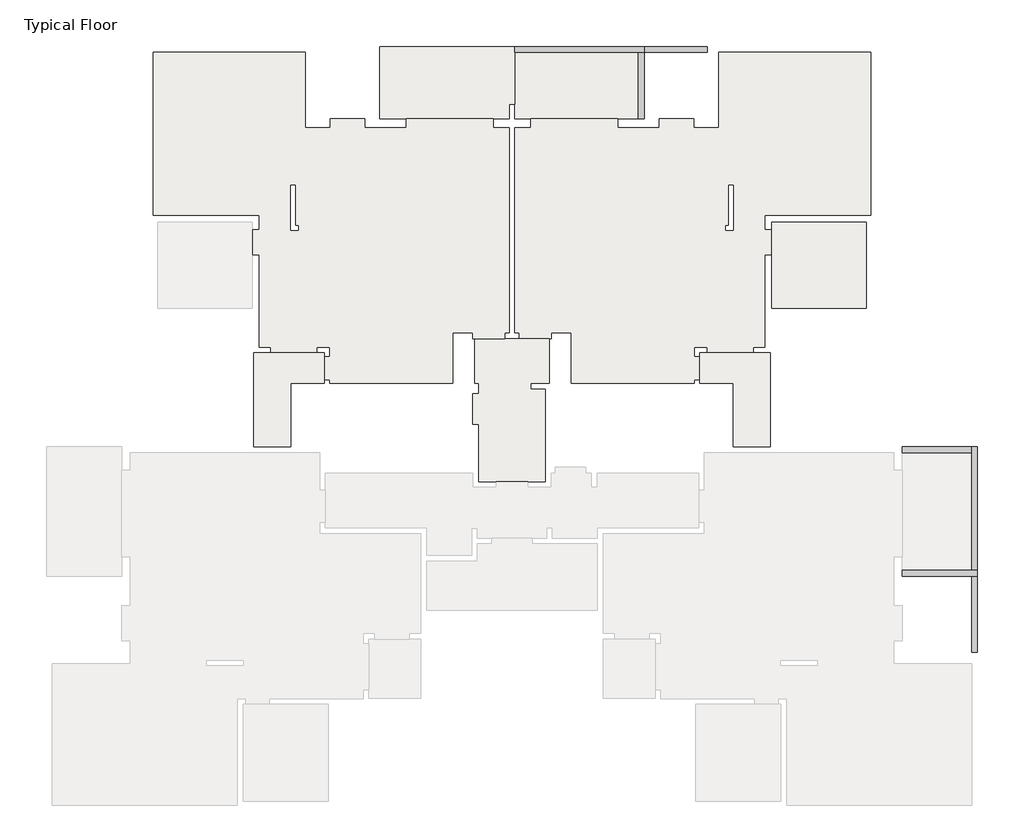
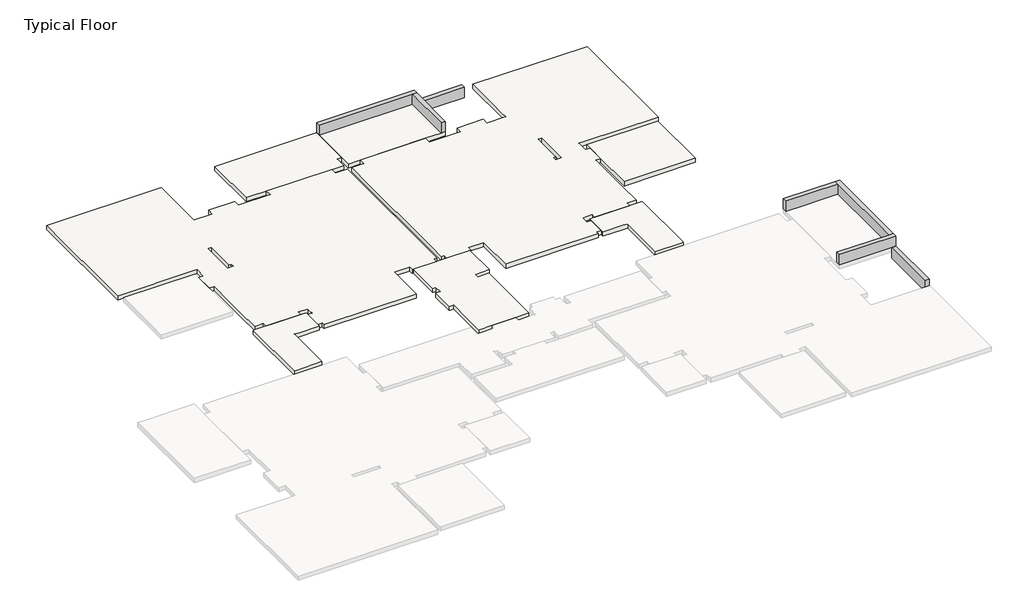
# One storey, part 2 of 2: 8 slabs, 7 beams.
"""IFC4 building model written with IfcOpenShell, lengths in millimetres."""

from ifc_helpers import new_model, si_unit, frame, origin, place, context, project, spatial, polyline, outline, extrude, faceted_brep, element, save

model = new_model("IFC4")

# Units and contexts
model_context = context("Model", 3, world=origin())
ifc_project = project(units=[si_unit("LENGTHUNIT", "METRE", prefix="MILLI")], contexts=[model_context])

# Site, building, storey
site = spatial("IfcSite", under=ifc_project)
building = spatial("IfcBuilding", under=site)
storey = spatial("IfcBuildingStorey", under=building, Name="Typical Floor", Elevation=3180.0)

# Beams
placement = place(None, origin())
element("IfcBeam", 1, ObjectType="Concrete Rectengular Beam : 20/50", at=placement, inside=storey, context=model_context, shape_type="Brep", body=[
    faceted_brep([(4727.4184919, 13929.1018304, 3680.0), (4727.4184919, 14129.1018304, 3680.0), (257.0516057, 14129.1018304, 3680.0), (257.0516057, 13929.1018304, 3680.0), (4527.4184919, 13929.1018304, 3680.0), (4727.4184919, 14129.1018304, 3180.0), (257.0516057, 14129.1018304, 3180.0), (4727.4184919, 13929.1018304, 3180.0), (4527.4184919, 13929.1018304, 3180.0), (257.0516057, 13929.1018304, 3180.0)], [[[0, 1, 2, 3, 4]], [[1, 5, 6, 2]], [[5, 7, 8, 9, 6]], [[7, 0, 4, 3, 9, 8]], [[3, 2, 6, 9]], [[1, 0, 7, 5]]]),
])
element("IfcBeam", 2, ObjectType="Concrete Rectengular Beam : 20/50", at=placement, inside=storey, context=model_context, shape_type="SweptSolid", body=[
    extrude(outline(polyline([(4727.4184919, 11629.007757), (4527.4184919, 11629.007757), (4527.4184919, 13929.1018304), (4727.4184919, 13929.1018304), (4727.4184919, 11629.007757)])), frame((0.0, 0.0, 3180.0), z_axis=(0.0, 0.0, 1.0), x_axis=(1.0, 0.0, 0.0)), (0.0, 0.0, 1.0), 500.0),
])
element("IfcBeam", 3, ObjectType="Concrete Rectengular Beam : 20/50", at=placement, inside=storey, context=model_context, shape_type="Brep", body=[
    faceted_brep([(16056.8164223, -4192.3939363, 3180.0), (16256.8164223, -4192.3939363, 3180.0), (16256.8164223, -4192.3939363, 2980.0), (16256.8164223, -4192.3939363, 2680.0), (16056.8164223, -4192.3939363, 2680.0), (16056.8164223, -6821.2744631, 3180.0), (16256.8164223, -6821.2744631, 3180.0), (16056.8164223, -6821.2744631, 2680.0), (16256.8164223, -6821.2744631, 2680.0)], [[[0, 1, 2, 3, 4]], [[1, 0, 5, 6]], [[0, 4, 7, 5]], [[4, 3, 8, 7]], [[3, 2, 1, 6, 8]], [[6, 5, 7, 8]]]),
])
element("IfcBeam", 4, ObjectType="Concrete Rectengular Beam : 20/50", at=placement, inside=storey, context=model_context, shape_type="Brep", body=[
    faceted_brep([(13657.004569, -4192.3939363, 3680.0), (13657.004569, -3992.3939363, 3680.0), (13657.004569, -3992.3939363, 3180.0), (13657.004569, -4192.3939363, 3180.0), (16256.8164223, -4192.3939363, 3680.0), (16256.8164223, -3992.3939363, 3680.0), (16056.8164223, -3992.3939363, 3680.0), (16256.8164223, -4192.3939363, 3180.0), (16056.8164223, -3992.3939363, 3180.0), (16256.8164223, -3992.3939363, 3180.0)], [[[0, 1, 2, 3]], [[1, 0, 4, 5, 6]], [[0, 3, 7, 4]], [[3, 2, 8, 9, 7]], [[2, 1, 6, 5, 9, 8]], [[5, 4, 7, 9]]]),
])
element("IfcBeam", 5, ObjectType="Concrete Rectengular Beam : 20/50", at=placement, inside=storey, context=model_context, shape_type="Brep", body=[
    faceted_brep([(16256.8164223, 279.007757, 3680.0), (16056.8164223, 279.007757, 3680.0), (16056.8164223, 79.007757, 3680.0), (16056.8164223, -3992.3939363, 3680.0), (16256.8164223, -3992.3939363, 3680.0), (16056.8164223, 279.007757, 3180.0), (16056.8164223, 79.007757, 3180.0), (16056.8164223, -3992.3939363, 3180.0), (16256.8164223, 279.007757, 3180.0), (16256.8164223, -3992.3939363, 3180.0)], [[[0, 1, 2, 3, 4]], [[1, 5, 6, 7, 3, 2]], [[5, 8, 9, 7, 6]], [[8, 0, 4, 9]], [[4, 3, 7, 9]], [[1, 0, 8, 5]]]),
])
element("IfcBeam", 6, ObjectType="Concrete Rectengular Beam : 20/50", at=placement, inside=storey, context=model_context, shape_type="SweptSolid", body=[
    extrude(outline(polyline([(13657.5690093, 79.007757), (13657.5690093, 279.007757), (16056.8164223, 279.007757), (16056.8164223, 79.007757), (13657.5690093, 79.007757)])), frame((0.0, 0.0, 3180.0), z_axis=(0.0, 0.0, 1.0), x_axis=(1.0, 0.0, 0.0)), (0.0, 0.0, 1.0), 500.0),
])
element("IfcBeam", 7, ObjectType="Concrete Rectengular Beam : 20/50", at=placement, inside=storey, context=model_context, shape_type="Brep", body=[
    faceted_brep([(4727.4184919, 13929.1018304, 2680.0), (4727.4184919, 13929.1018304, 3180.0), (4727.4184919, 14129.1018304, 3180.0), (4727.4184919, 14129.1018304, 2980.0), (4727.4184919, 14129.1018304, 2680.0), (6907.5690093, 13929.1018304, 3180.0), (6907.5690093, 13929.3370139, 3180.0), (6907.5690093, 14129.1018304, 3180.0), (6907.5690093, 14129.1018304, 2680.0), (6907.5690093, 13929.1018304, 2680.0)], [[[0, 1, 2, 3, 4]], [[2, 1, 5, 6, 7]], [[4, 3, 2, 7, 8]], [[0, 4, 8, 9]], [[1, 0, 9, 5]], [[5, 9, 8, 7, 6]]]),
])

# Slabs
element("IfcSlab", 8, ObjectType="20", at=placement, inside=storey, context=model_context, shape_type="Brep", body=[
    faceted_brep([(-6993.4657979, 11328.25517, 2980.0), (-6133.4657979, 11328.25517, 2980.0), (-6133.4657979, 11628.25517, 2980.0), (-4944.5946784, 11628.25517, 2980.0), (-4944.5946784, 11329.007757, 2980.0), (-3494.6887518, 11329.007757, 2980.0), (-3494.6887518, 11629.007757, 2980.0), (-491.1610001, 11629.007757, 2980.0), (-491.1610001, 11329.007757, 2980.0), (57.0516057, 11329.007757, 2980.0), (57.0516057, 4229.007757, 2980.0), (-93.2306144, 4229.007757, 2980.0), (-93.2306144, 4029.007757, 2980.0), (-1133.7398977, 4029.007757, 2980.0), (-1193.8891281, 4029.007757, 2980.0), (-1193.8891281, 4228.6785002, 2980.0), (-1894.500605, 4228.6785002, 2980.0), (-1894.500605, 4028.6785002, 2980.0), (-1894.500605, 2479.2899772, 2980.0), (-6144.7357885, 2479.2899772, 2980.0), (-6144.7357885, 2597.8224325, 2980.0), (-6344.7357885, 2597.8224325, 2980.0), (-6344.7357885, 3397.9165059, 2980.0), (-6144.7357885, 3397.9165059, 2980.0), (-6144.7357885, 3529.1488671, 2980.0), (-6144.7357885, 3729.1488671, 2980.0), (-6593.4657979, 3729.1488671, 2980.0), (-6593.4657979, 3529.1488671, 2980.0), (-8193.6539446, 3529.1488671, 2980.0), (-8193.6539446, 3729.1488671, 2980.0), (-8593.7009813, 3729.1488671, 2980.0), (-8593.7009813, 4828.7725736, 2980.0), (-8593.7009813, 6932.7236554, 2980.0), (-8823.7009813, 6932.7236554, 2980.0), (-8823.7009813, 7785.2636366, 2980.0), (-8593.7009813, 7785.2636366, 2980.0), (-8593.7009813, 8285.2636366, 2980.0), (-8823.7009813, 8285.2636366, 2980.0), (-12243.8891281, 8285.2636366, 2980.0), (-12243.8891281, 13929.3370139, 2980.0), (-6993.4657979, 13929.3370139, 2980.0), (-6993.4657979, 11628.25517, 2980.0), (-7340.9258167, 9328.7725736, 2980.0), (-7490.9258167, 9328.7725736, 2980.0), (-7490.9258167, 7927.5496197, 2980.0), (-7490.9258167, 7777.5496197, 2980.0), (-7241.1610001, 7777.5496197, 2980.0), (-7241.1610001, 7927.5496197, 2980.0), (-7340.9258167, 7927.5496197, 2980.0), (-6133.4657979, 11328.25517, 3180.0), (-6993.4657979, 11328.25517, 3180.0), (-6993.4657979, 11628.25517, 3180.0), (-6993.4657979, 13929.3370139, 3180.0), (-12243.8891281, 13929.3370139, 3180.0), (-12243.8891281, 8285.2636366, 3180.0), (-8823.7009813, 8285.2636366, 3180.0), (-8593.7009813, 8285.2636366, 3180.0), (-8593.7009813, 7785.2636366, 3180.0), (-8823.7009813, 7785.2636366, 3180.0), (-8823.7009813, 6932.7236554, 3180.0), (-8593.7009813, 6932.7236554, 3180.0), (-8593.7009813, 4828.7725736, 3180.0), (-8593.7009813, 3729.1488671, 3180.0), (-8193.6539446, 3729.1488671, 3180.0), (-8193.6539446, 3529.1488671, 3180.0), (-6593.4657979, 3529.1488671, 3180.0), (-6593.4657979, 3729.1488671, 3180.0), (-6144.7357885, 3729.1488671, 3180.0), (-6144.7357885, 3529.1488671, 3180.0), (-6144.7357885, 3397.9165059, 3180.0), (-6344.7357885, 3397.9165059, 3180.0), (-6344.7357885, 2597.8224325, 3180.0), (-6144.7357885, 2597.8224325, 3180.0), (-6144.7357885, 2479.2899772, 3180.0), (-1894.500605, 2479.2899772, 3180.0), (-1894.500605, 4028.6785002, 3180.0), (-1894.500605, 4228.6785002, 3180.0), (-1193.8891281, 4228.6785002, 3180.0), (-1193.8891281, 4029.007757, 3180.0), (-1133.7398977, 4029.007757, 3180.0), (-93.2306144, 4029.007757, 3180.0), (-93.2306144, 4229.007757, 3180.0), (57.0516057, 4229.007757, 3180.0), (57.0516057, 11329.007757, 3180.0), (-491.1610001, 11329.007757, 3180.0), (-491.1610001, 11629.007757, 3180.0), (-3494.6887518, 11629.007757, 3180.0), (-3494.6887518, 11329.007757, 3180.0), (-4944.5946784, 11329.007757, 3180.0), (-4944.5946784, 11628.25517, 3180.0), (-6133.4657979, 11628.25517, 3180.0), (-7490.9258167, 9328.7725736, 3180.0), (-7340.9258167, 9328.7725736, 3180.0), (-7340.9258167, 7927.5496197, 3180.0), (-7241.1610001, 7927.5496197, 3180.0), (-7241.1610001, 7777.5496197, 3180.0), (-7490.9258167, 7777.5496197, 3180.0), (-7490.9258167, 7927.5496197, 3180.0)], [[[0, 1, 2, 3, 4, 5, 6, 7, 8, 9, 10, 11, 12, 13, 14, 15, 16, 17, 18, 19, 20, 21, 22, 23, 24, 25, 26, 27, 28, 29, 30, 31, 32, 33, 34, 35, 36, 37, 38, 39, 40, 41], [42, 43, 44, 45, 46, 47, 48]], [[49, 50, 51, 52, 53, 54, 55, 56, 57, 58, 59, 60, 61, 62, 63, 64, 65, 66, 67, 68, 69, 70, 71, 72, 73, 74, 75, 76, 77, 78, 79, 80, 81, 82, 83, 84, 85, 86, 87, 88, 89, 90], [91, 92, 93, 94, 95, 96, 97]], [[50, 0, 41, 40, 52, 51]], [[1, 0, 50, 49]], [[2, 1, 49, 90]], [[3, 2, 90, 89]], [[4, 3, 89, 88]], [[5, 4, 88, 87]], [[6, 5, 87, 86]], [[7, 6, 86, 85]], [[8, 7, 85, 84]], [[9, 8, 84, 83]], [[10, 9, 83, 82]], [[11, 10, 82, 81]], [[12, 11, 81, 80]], [[14, 13, 12, 80, 79, 78]], [[15, 14, 78, 77]], [[16, 15, 77, 76]], [[16, 76, 75, 74, 18, 17]], [[19, 18, 74, 73]], [[20, 19, 73, 72]], [[21, 20, 72, 71]], [[22, 21, 71, 70]], [[23, 22, 70, 69]], [[23, 69, 68, 67, 25, 24]], [[26, 25, 67, 66]], [[27, 26, 66, 65]], [[28, 27, 65, 64]], [[29, 28, 64, 63]], [[30, 29, 63, 62]], [[30, 62, 61, 60, 32, 31]], [[33, 32, 60, 59]], [[34, 33, 59, 58]], [[35, 34, 58, 57]], [[36, 35, 57, 56]], [[36, 56, 55, 54, 38, 37]], [[39, 38, 54, 53]], [[40, 39, 53, 52]], [[43, 42, 92, 91]], [[43, 91, 97, 96, 45, 44]], [[46, 45, 96, 95]], [[47, 46, 95, 94]], [[48, 47, 94, 93]], [[42, 48, 93, 92]]]),
])
element("IfcSlab", 9, ObjectType="20", at=placement, inside=storey, context=model_context, shape_type="Brep", body=[
    faceted_brep([(57.0516057, 12129.1018304, 2980.0), (57.0516057, 11629.007757, 2980.0), (-491.1610001, 11629.007757, 2980.0), (-3494.6887518, 11629.007757, 2980.0), (-4413.3152805, 11629.007757, 2980.0), (-4413.3152805, 14129.1018304, 2980.0), (57.0516057, 14129.1018304, 2980.0), (257.0516057, 14129.1018304, 2980.0), (257.0516057, 13929.1018304, 2980.0), (257.0516057, 12129.1018304, 2980.0), (57.0516057, 11629.007757, 3180.0), (57.0516057, 12129.1018304, 3180.0), (257.0516057, 12129.1018304, 3180.0), (257.0516057, 13929.1018304, 3180.0), (257.0516057, 14129.1018304, 3180.0), (57.0516057, 14129.1018304, 3180.0), (-4213.3152805, 14129.1018304, 3180.0), (-4413.3152805, 14129.1018304, 3180.0), (-4413.3152805, 13929.1018304, 3180.0), (-4413.3152805, 11629.007757, 3180.0), (-4213.3152805, 11629.007757, 3180.0), (-3494.6887518, 11629.007757, 3180.0), (-491.1610001, 11629.007757, 3180.0)], [[[0, 1, 2, 3, 4, 5, 6, 7, 8, 9]], [[10, 11, 12, 13, 14, 15, 16, 17, 18, 19, 20, 21, 22]], [[1, 0, 11, 10]], [[1, 10, 22, 21, 20, 19, 4, 3, 2]], [[5, 4, 19, 18, 17]], [[6, 5, 17, 16, 15]], [[7, 6, 15, 14]], [[8, 7, 14, 13]], [[9, 8, 13, 12]], [[0, 9, 12, 11]]]),
])
element("IfcSlab", 10, ObjectType="20", at=placement, inside=storey, context=model_context, shape_type="Brep", body=[
    faceted_brep([(6447.5690093, 11328.25517, 2980.0), (7307.5690093, 11328.25517, 2980.0), (7307.5690093, 11628.25517, 2980.0), (7307.5690093, 13929.3370139, 2980.0), (12557.9923395, 13929.3370139, 2980.0), (12557.9923395, 8285.2636366, 2980.0), (9137.8041927, 8285.2636366, 2980.0), (8907.8041927, 8285.2636366, 2980.0), (8907.8041927, 7785.2636366, 2980.0), (9137.8041927, 7785.2636366, 2980.0), (9137.8041927, 6932.7236554, 2980.0), (8907.8041927, 6932.7236554, 2980.0), (8907.8041927, 4828.7725736, 2980.0), (8907.8041927, 3729.1488671, 2980.0), (8507.757156, 3729.1488671, 2980.0), (8507.757156, 3529.1488671, 2980.0), (6907.5690093, 3529.1488671, 2980.0), (6907.5690093, 3729.1488671, 2980.0), (6458.8389999, 3729.1488671, 2980.0), (6458.8389999, 3529.1488671, 2980.0), (6458.8389999, 3397.9165059, 2980.0), (6658.8389999, 3397.9165059, 2980.0), (6658.8389999, 2597.8224325, 2980.0), (6458.8389999, 2597.8224325, 2980.0), (6458.8389999, 2479.2899772, 2980.0), (2208.6038164, 2479.2899772, 2980.0), (2208.6038164, 4028.6785002, 2980.0), (2208.6038164, 4228.6785002, 2980.0), (1507.9923395, 4228.6785002, 2980.0), (1507.9923395, 4029.007757, 2980.0), (1446.2601023, 4029.007757, 2980.0), (407.3338258, 4029.007757, 2980.0), (407.3338258, 4229.007757, 2980.0), (257.0516057, 4229.007757, 2980.0), (257.0516057, 11329.007757, 2980.0), (806.3460554, 11329.007757, 2980.0), (806.3460554, 11629.007757, 2980.0), (3808.7919632, 11629.007757, 2980.0), (3808.7919632, 11329.007757, 2980.0), (5258.6978898, 11329.007757, 2980.0), (5258.6978898, 11628.25517, 2980.0), (6447.5690093, 11628.25517, 2980.0), (7805.0290281, 9328.7725736, 2980.0), (7655.0290281, 9328.7725736, 2980.0), (7655.0290281, 7927.5496197, 2980.0), (7555.2642115, 7927.5496197, 2980.0), (7555.2642115, 7777.5496197, 2980.0), (7805.0290281, 7777.5496197, 2980.0), (7805.0290281, 7927.5496197, 2980.0), (7307.5690093, 11328.25517, 3180.0), (6447.5690093, 11328.25517, 3180.0), (6447.5690093, 11628.25517, 3180.0), (5258.6978898, 11628.25517, 3180.0), (5258.6978898, 11329.007757, 3180.0), (3808.7919632, 11329.007757, 3180.0), (3808.7919632, 11629.007757, 3180.0), (806.3460554, 11629.007757, 3180.0), (806.3460554, 11329.007757, 3180.0), (257.0516057, 11329.007757, 3180.0), (257.0516057, 4229.007757, 3180.0), (407.3338258, 4229.007757, 3180.0), (407.3338258, 4029.007757, 3180.0), (1446.2601023, 4029.007757, 3180.0), (1507.9923395, 4029.007757, 3180.0), (1507.9923395, 4228.6785002, 3180.0), (2208.6038164, 4228.6785002, 3180.0), (2208.6038164, 4028.6785002, 3180.0), (2208.6038164, 2479.2899772, 3180.0), (6458.8389999, 2479.2899772, 3180.0), (6458.8389999, 2597.8224325, 3180.0), (6658.8389999, 2597.8224325, 3180.0), (6658.8389999, 3397.9165059, 3180.0), (6458.8389999, 3397.9165059, 3180.0), (6458.8389999, 3529.1488671, 3180.0), (6458.8389999, 3729.1488671, 3180.0), (6907.5690093, 3729.1488671, 3180.0), (6907.5690093, 3529.1488671, 3180.0), (8507.757156, 3529.1488671, 3180.0), (8507.757156, 3729.1488671, 3180.0), (8907.8041927, 3729.1488671, 3180.0), (8907.8041927, 4828.7725736, 3180.0), (8907.8041927, 6932.7236554, 3180.0), (9137.8041927, 6932.7236554, 3180.0), (9137.8041927, 7785.2636366, 3180.0), (8907.8041927, 7785.2636366, 3180.0), (8907.8041927, 8285.2636366, 3180.0), (9137.8041927, 8285.2636366, 3180.0), (12557.9923395, 8285.2636366, 3180.0), (12557.9923395, 13929.3370139, 3180.0), (7307.5690093, 13929.3370139, 3180.0), (7307.5690093, 11628.25517, 3180.0), (7655.0290281, 9328.7725736, 3180.0), (7805.0290281, 9328.7725736, 3180.0), (7805.0290281, 7927.5496197, 3180.0), (7805.0290281, 7777.5496197, 3180.0), (7555.2642115, 7777.5496197, 3180.0), (7555.2642115, 7927.5496197, 3180.0), (7655.0290281, 7927.5496197, 3180.0)], [[[0, 1, 2, 3, 4, 5, 6, 7, 8, 9, 10, 11, 12, 13, 14, 15, 16, 17, 18, 19, 20, 21, 22, 23, 24, 25, 26, 27, 28, 29, 30, 31, 32, 33, 34, 35, 36, 37, 38, 39, 40, 41], [42, 43, 44, 45, 46, 47, 48]], [[49, 50, 51, 52, 53, 54, 55, 56, 57, 58, 59, 60, 61, 62, 63, 64, 65, 66, 67, 68, 69, 70, 71, 72, 73, 74, 75, 76, 77, 78, 79, 80, 81, 82, 83, 84, 85, 86, 87, 88, 89, 90], [91, 92, 93, 94, 95, 96, 97]], [[1, 49, 90, 89, 3, 2]], [[1, 0, 50, 49]], [[0, 41, 51, 50]], [[41, 40, 52, 51]], [[40, 39, 53, 52]], [[39, 38, 54, 53]], [[38, 37, 55, 54]], [[55, 37, 36, 56]], [[34, 58, 57, 35]], [[34, 33, 59, 58]], [[33, 32, 60, 59]], [[32, 31, 61, 60]], [[31, 30, 29, 63, 62, 61]], [[29, 28, 64, 63]], [[28, 27, 65, 64]], [[25, 67, 66, 65, 27, 26]], [[25, 24, 68, 67]], [[24, 23, 69, 68]], [[23, 22, 70, 69]], [[22, 21, 71, 70]], [[21, 20, 72, 71]], [[18, 74, 73, 72, 20, 19]], [[18, 17, 75, 74]], [[17, 16, 76, 75]], [[16, 15, 77, 76]], [[15, 14, 78, 77]], [[14, 13, 79, 78]], [[11, 81, 80, 79, 13, 12]], [[11, 10, 82, 81]], [[10, 9, 83, 82]], [[9, 8, 84, 83]], [[8, 7, 85, 84]], [[5, 87, 86, 85, 7, 6]], [[5, 4, 88, 87]], [[4, 3, 89, 88]], [[43, 42, 92, 91]], [[47, 94, 93, 92, 42, 48]], [[47, 46, 95, 94]], [[46, 45, 96, 95]], [[45, 44, 97, 96]], [[44, 43, 91, 97]], [[35, 57, 56, 36]]]),
])
element("IfcSlab", 11, ObjectType="20", at=placement, inside=storey, context=model_context, shape_type="Brep", body=[
    faceted_brep([(12407.9923395, 8055.2636366, 2980.0), (12407.9923395, 5078.7725736, 2980.0), (9137.8041927, 5078.7725736, 2980.0), (9137.8041927, 6932.7236554, 2980.0), (9137.8041927, 7785.2636366, 2980.0), (9137.8041927, 8055.2636366, 2980.0), (12407.9923395, 5078.7725736, 3180.0), (12407.9923395, 8055.2636366, 3180.0), (9137.8041927, 8055.2636366, 3180.0), (9137.8041927, 7785.2636366, 3180.0), (9137.8041927, 6932.7236554, 3180.0), (9137.8041927, 5078.7725736, 3180.0)], [[[0, 1, 2, 3, 4, 5]], [[6, 7, 8, 9, 10, 11]], [[1, 6, 11, 2]], [[1, 0, 7, 6]], [[7, 0, 5, 8]], [[8, 5, 4, 3, 2, 11, 10, 9]]]),
])
element("IfcSlab", 12, ObjectType="20", at=placement, inside=storey, context=model_context, shape_type="Brep", body=[
    faceted_brep([(1446.2601023, 4029.007757, 2980.0), (1446.2601023, 2479.2899772, 2980.0), (806.3460554, 2479.2899772, 2980.0), (806.3460554, 2279.2899772, 2980.0), (1309.0271466, 2279.2899772, 2980.0), (1309.0271466, -921.133353, 2980.0), (707.8982661, -921.133353, 2980.0), (-393.7950547, -921.133353, 2980.0), (-994.9239352, -921.133353, 2980.0), (-994.9239352, 1067.4837683, 2980.0), (-1194.9239352, 1067.4837683, 2980.0), (-1194.9239352, 2127.9259132, 2980.0), (-994.9239352, 2127.9259132, 2980.0), (-994.9239352, 2479.2899772, 2980.0), (-1133.7398977, 2479.2899772, 2980.0), (-1133.7398977, 4020.7370491, 2980.0), (-1133.7398977, 4029.007757, 2980.0), (-93.2306144, 4029.007757, 2980.0), (407.3338258, 4029.007757, 2980.0), (1446.2601023, 2479.2899772, 3180.0), (1446.2601023, 4029.007757, 3180.0), (407.3338258, 4029.007757, 3180.0), (-93.2306144, 4029.007757, 3180.0), (-1133.7398977, 4029.007757, 3180.0), (-1133.7398977, 4020.7370491, 3180.0), (-1133.7398977, 2479.2899772, 3180.0), (-994.9239352, 2479.2899772, 3180.0), (-994.9239352, 2127.9259132, 3180.0), (-1194.9239352, 2127.9259132, 3180.0), (-1194.9239352, 1067.4837683, 3180.0), (-994.9239352, 1067.4837683, 3180.0), (-994.9239352, -921.133353, 3180.0), (-393.7950547, -921.133353, 3180.0), (707.8982661, -921.133353, 3180.0), (1309.0271466, -921.133353, 3180.0), (1309.0271466, 2279.2899772, 3180.0), (806.3460554, 2279.2899772, 3180.0), (806.3460554, 2479.2899772, 3180.0)], [[[0, 1, 2, 3, 4, 5, 6, 7, 8, 9, 10, 11, 12, 13, 14, 15, 16, 17, 18]], [[19, 20, 21, 22, 23, 24, 25, 26, 27, 28, 29, 30, 31, 32, 33, 34, 35, 36, 37]], [[20, 0, 18, 17, 16, 23, 22, 21]], [[1, 0, 20, 19]], [[2, 1, 19, 37]], [[3, 2, 37, 36]], [[4, 3, 36, 35]], [[5, 4, 35, 34]], [[5, 34, 33, 32, 31, 8, 7, 6]], [[9, 8, 31, 30]], [[10, 9, 30, 29]], [[11, 10, 29, 28]], [[12, 11, 28, 27]], [[13, 12, 27, 26]], [[14, 13, 26, 25]], [[15, 14, 25, 24]], [[16, 15, 24, 23]]]),
])
element("IfcSlab", 13, ObjectType="20", at=placement, inside=storey, context=model_context, shape_type="Brep", body=[
    faceted_brep([(9086.6847195, 3529.1488671, 2980.0), (9086.6847195, 279.007757, 2980.0), (7807.1456791, 279.007757, 2980.0), (7807.1456791, 2479.2899772, 2980.0), (7607.1456791, 2479.2899772, 2980.0), (6658.8389999, 2479.2899772, 2980.0), (6658.8389999, 2597.8224325, 2980.0), (6658.8389999, 3397.9165059, 2980.0), (6658.8389999, 3529.1488671, 2980.0), (6907.5690093, 3529.1488671, 2980.0), (8507.757156, 3529.1488671, 2980.0), (9086.6847195, 279.007757, 3180.0), (9086.6847195, 3529.1488671, 3180.0), (8986.6847195, 3529.1488671, 3180.0), (8507.757156, 3529.1488671, 3180.0), (6907.5690093, 3529.1488671, 3180.0), (6658.8389999, 3529.1488671, 3180.0), (6658.8389999, 3397.9165059, 3180.0), (6658.8389999, 2597.8224325, 3180.0), (6658.8389999, 2479.2899772, 3180.0), (7607.1456791, 2479.2899772, 3180.0), (7807.1456791, 2479.2899772, 3180.0), (7807.1456791, 279.007757, 3180.0), (8986.6847195, 279.007757, 3180.0)], [[[0, 1, 2, 3, 4, 5, 6, 7, 8, 9, 10]], [[11, 12, 13, 14, 15, 16, 17, 18, 19, 20, 21, 22, 23]], [[1, 0, 12, 11]], [[2, 1, 11, 23, 22]], [[3, 2, 22, 21]], [[3, 21, 20, 19, 5, 4]], [[5, 19, 18, 17, 16, 8, 7, 6]], [[8, 16, 15, 14, 13, 12, 0, 10, 9]]]),
])
element("IfcSlab", 14, ObjectType="20", at=placement, inside=storey, context=model_context, shape_type="Brep", body=[
    faceted_brep([(-8774.1337189, 279.007757, 2980.0), (-8774.1337189, 3529.1488671, 2980.0), (-8193.6539446, 3529.1488671, 2980.0), (-6593.4657979, 3529.1488671, 2980.0), (-6344.7357885, 3529.1488671, 2980.0), (-6344.7357885, 3397.9165059, 2980.0), (-6344.7357885, 2597.8224325, 2980.0), (-6344.7357885, 2479.2899772, 2980.0), (-7293.0424677, 2479.2899772, 2980.0), (-7493.0424677, 2479.2899772, 2980.0), (-7493.0424677, 279.007757, 2980.0), (-8774.1337189, 3529.1488671, 3180.0), (-8774.1337189, 279.007757, 3180.0), (-8674.1337189, 279.007757, 3180.0), (-7493.0424677, 279.007757, 3180.0), (-7493.0424677, 2479.2899772, 3180.0), (-7293.0424677, 2479.2899772, 3180.0), (-6344.7357885, 2479.2899772, 3180.0), (-6344.7357885, 2597.8224325, 3180.0), (-6344.7357885, 3397.9165059, 3180.0), (-6344.7357885, 3529.1488671, 3180.0), (-6593.4657979, 3529.1488671, 3180.0), (-8193.6539446, 3529.1488671, 3180.0), (-8674.1337189, 3529.1488671, 3180.0)], [[[0, 1, 2, 3, 4, 5, 6, 7, 8, 9, 10]], [[11, 12, 13, 14, 15, 16, 17, 18, 19, 20, 21, 22, 23]], [[1, 0, 12, 11]], [[0, 10, 14, 13, 12]], [[10, 9, 15, 14]], [[7, 17, 16, 15, 9, 8]], [[4, 20, 19, 18, 17, 7, 6, 5]], [[20, 4, 3, 2, 1, 11, 23, 22, 21]]]),
])
element("IfcSlab", 15, ObjectType="20", at=placement, inside=storey, context=model_context, shape_type="Brep", body=[
    faceted_brep([(257.0516057, 11629.007757, 2980.0), (257.0516057, 12129.1018304, 2980.0), (257.0516057, 14129.1018304, 2980.0), (4727.4184919, 14129.1018304, 2980.0), (4727.4184919, 11629.007757, 2980.0), (3808.7919632, 11629.007757, 2980.0), (806.3460554, 11629.007757, 2980.0), (805.2642115, 11629.007757, 2980.0), (257.0516057, 14129.1018304, 3180.0), (257.0516057, 13929.1018304, 3180.0), (257.0516057, 12129.1018304, 3180.0), (257.0516057, 11629.007757, 3180.0), (805.2642115, 11629.007757, 3180.0), (806.3460554, 11629.007757, 3180.0), (3808.7919632, 11629.007757, 3180.0), (4527.4184919, 11629.007757, 3180.0), (4727.4184919, 11629.007757, 3180.0), (4727.4184919, 13929.1018304, 3180.0), (4727.4184919, 14129.1018304, 3180.0)], [[[0, 1, 2, 3, 4, 5, 6, 7]], [[8, 9, 10, 11, 12, 13, 14, 15, 16, 17, 18]], [[2, 1, 0, 11, 10, 9, 8]], [[4, 16, 15, 14, 13, 12, 11, 0, 7, 6, 5]], [[4, 3, 18, 17, 16]], [[3, 2, 8, 18]]]),
])

save(model, "model.ifc")

# Revit data of these elements
# Type "Concrete Rectengular Beam : 20/50"
#   Type IfcGUID = "1zn3TUKgbD69x5FAYjkT3O"
#   Length [instance default] = 152.4 cm
#   b = 20 cm
#   h = 50 cm
#   Structural Material [instance default] = Concrete
#   Assembly Code = ""
# Type "20"
#   Type IfcGUID = "1zn3TUKgbD69x5FAYjkTF1"
#   Function = 0
#   Layers, outside or top first: 20 cm "Concrete" (function 1)
# Element 1 (IfcBeam, "Concrete Rectengular Beam : 20/50")
#   IfcGUID = "3brXM_Qu1DvOaG$o2DBD19"
#   Comments = ""
#   Mark = "B13"
#   SOFiSTiK_AMG_Comments = ""
#   SOFiSTiK_AMG_Scheduled = yes
#   SOFiSTiK_AMG_Adjusted = yes
#   Structural Material = Concrete
#   Phase Created = New Construction
#   Materials on its faces: "Concrete"
# Element 2 (IfcBeam, "Concrete Rectengular Beam : 20/50")
#   IfcGUID = "3brXM_Qu1DvOaG$o2DBD1B"
#   Comments = ""
#   Mark = "B14"
#   SOFiSTiK_AMG_Comments = ""
#   SOFiSTiK_AMG_Scheduled = yes
#   SOFiSTiK_AMG_Adjusted = yes
#   Structural Material = Concrete
#   Phase Created = New Construction
#   Materials on its faces: "Concrete"
# Element 3 (IfcBeam, "Concrete Rectengular Beam : 20/50")
#   IfcGUID = "3brXM_Qu1DvOaG$o2DBD1D"
#   Comments = ""
#   Mark = "B15"
#   SOFiSTiK_AMG_Comments = ""
#   SOFiSTiK_AMG_Scheduled = yes
#   SOFiSTiK_AMG_Adjusted = yes
#   Structural Material = Concrete
#   Phase Created = New Construction
#   Materials on its faces: "Concrete"
# Element 4 (IfcBeam, "Concrete Rectengular Beam : 20/50")
#   IfcGUID = "3brXM_Qu1DvOaG$o2DBD4K"
#   Comments = ""
#   Mark = "B16"
#   SOFiSTiK_AMG_Comments = ""
#   SOFiSTiK_AMG_Scheduled = yes
#   SOFiSTiK_AMG_Adjusted = yes
#   Structural Material = Concrete
#   Phase Created = New Construction
#   Materials on its faces: "Concrete"
# Element 5 (IfcBeam, "Concrete Rectengular Beam : 20/50")
#   IfcGUID = "3brXM_Qu1DvOaG$o2DBD4M"
#   Comments = ""
#   Mark = "B17"
#   SOFiSTiK_AMG_Comments = ""
#   SOFiSTiK_AMG_Scheduled = yes
#   SOFiSTiK_AMG_Adjusted = yes
#   Structural Material = Concrete
#   Phase Created = New Construction
#   Materials on its faces: "Concrete"
# Element 6 (IfcBeam, "Concrete Rectengular Beam : 20/50")
#   IfcGUID = "3brXM_Qu1DvOaG$o2DBD4O"
#   Comments = ""
#   Mark = "B18"
#   SOFiSTiK_AMG_Comments = ""
#   SOFiSTiK_AMG_Scheduled = yes
#   SOFiSTiK_AMG_Adjusted = yes
#   Structural Material = Concrete
#   Phase Created = New Construction
#   Materials on its faces: "Concrete"
# Element 7 (IfcBeam, "Concrete Rectengular Beam : 20/50")
#   IfcGUID = "3brXM_Qu1DvOaG$o2DBD5p"
#   Comments = ""
#   Mark = "B19"
#   SOFiSTiK_AMG_Comments = ""
#   SOFiSTiK_AMG_Scheduled = yes
#   SOFiSTiK_AMG_Adjusted = yes
#   Structural Material = Concrete
#   Phase Created = New Construction
#   Materials on its faces: "Concrete"
# Element 8 (IfcSlab, "20")
#   IfcGUID = "1e7LVzuKbECxrDX1g1kJ0y"
#   Mark = "S1"
#   SOFiSTiK_AMG_Comments = ""
#   Height Offset From Level = 0 cm
#   built-in parameter 1001954 = 1
#   SOFiSTiK_AMG_Scheduled = yes
#   SOFiSTiK_AMG_Adjusted = yes
#   Phase Created = New Construction
#   Materials on its faces: "Concrete"
# Element 9 (IfcSlab, "20")
#   IfcGUID = "3brXM_Qu1DvOaG$o2DBDVq"
#   Mark = "S6"
#   SOFiSTiK_AMG_Comments = ""
#   Height Offset From Level = 0 cm
#   built-in parameter 1001954 = 1
#   SOFiSTiK_AMG_Scheduled = yes
#   SOFiSTiK_AMG_Adjusted = yes
#   Phase Created = New Construction
#   Materials on its faces: "Concrete"
# Element 10 (IfcSlab, "20")
#   IfcGUID = "3brXM_Qu1DvOaG$o2DBD2n"
#   Mark = "S7"
#   SOFiSTiK_AMG_Comments = ""
#   built-in parameter 1001955 = 3.14159 (stored number, unit not read)
#   Height Offset From Level = 0 cm
#   built-in parameter 1001954 = 1
#   SOFiSTiK_AMG_Scheduled = yes
#   SOFiSTiK_AMG_Adjusted = yes
#   Phase Created = New Construction
#   Materials on its faces: "Concrete"
# Element 11 (IfcSlab, "20")
#   IfcGUID = "3brXM_Qu1DvOaG$o2DBD3t"
#   Mark = "S8"
#   SOFiSTiK_AMG_Comments = ""
#   built-in parameter 1001955 = 3.14159 (stored number, unit not read)
#   Height Offset From Level = 0 cm
#   built-in parameter 1001954 = 1
#   SOFiSTiK_AMG_Scheduled = yes
#   SOFiSTiK_AMG_Adjusted = yes
#   Phase Created = New Construction
#   Materials on its faces: "Concrete"
# Element 12 (IfcSlab, "20")
#   IfcGUID = "3brXM_Qu1DvOaG$o2DB3sh"
#   Mark = "S14"
#   SOFiSTiK_AMG_Comments = ""
#   built-in parameter 1001955 = 1.5708 (stored number, unit not read)
#   Height Offset From Level = 0 cm
#   built-in parameter 1001954 = 1
#   SOFiSTiK_AMG_Scheduled = yes
#   SOFiSTiK_AMG_Adjusted = yes
#   Phase Created = New Construction
#   Materials on its faces: "Concrete"
# Element 13 (IfcSlab, "20")
#   IfcGUID = "3brXM_Qu1DvOaG$o2DB3is"
#   Mark = "S15"
#   SOFiSTiK_AMG_Comments = ""
#   Height Offset From Level = 0 cm
#   built-in parameter 1001954 = 1
#   SOFiSTiK_AMG_Scheduled = yes
#   SOFiSTiK_AMG_Adjusted = yes
#   Phase Created = New Construction
#   Materials on its faces: "Concrete"
# Element 14 (IfcSlab, "20")
#   IfcGUID = "3brXM_Qu1DvOaG$o2DB3MT"
#   Mark = "S16"
#   SOFiSTiK_AMG_Comments = ""
#   built-in parameter 1001955 = 3.14159 (stored number, unit not read)
#   Height Offset From Level = 0 cm
#   built-in parameter 1001954 = 1
#   SOFiSTiK_AMG_Scheduled = yes
#   SOFiSTiK_AMG_Adjusted = yes
#   Phase Created = New Construction
#   Materials on its faces: "Concrete"
# Element 15 (IfcSlab, "20")
#   IfcGUID = "3brXM_Qu1DvOaG$o2DB3Qg"
#   Mark = "S19"
#   SOFiSTiK_AMG_Comments = ""
#   built-in parameter 1001955 = 3.14159 (stored number, unit not read)
#   Height Offset From Level = 0 cm
#   built-in parameter 1001954 = 1
#   SOFiSTiK_AMG_Scheduled = yes
#   SOFiSTiK_AMG_Adjusted = yes
#   Phase Created = New Construction
#   Materials on its faces: "Concrete"
# Materials
#   "Concrete": class "Concrete", colour RGB 192 192 192, transparency 0, Keynote = "01000", Description = "Cast-in-place concrete", Cost = 0
